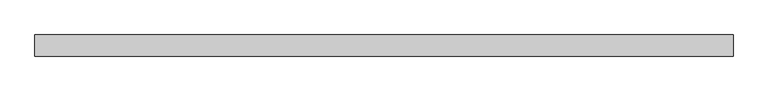
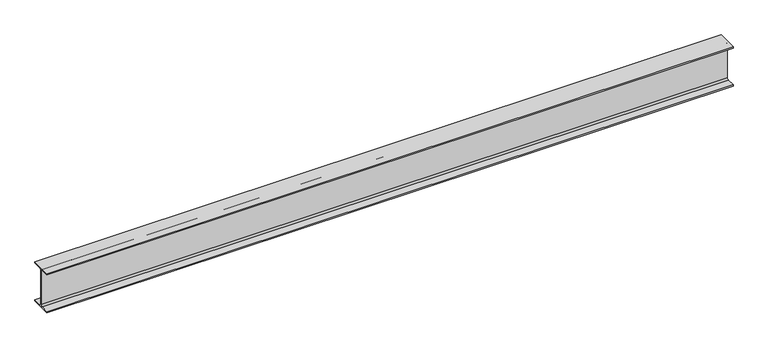
"""IFC4 building model written with IfcOpenShell, lengths in millimetres: beam geometry, 0912_Steel Framing_H-KSD3502 : H_SB_AR_S02_H-350x175x7x11_Platform."""

from ifc_helpers import new_model, si_unit, point, frame, frame_2d, origin, place, context, project, spatial, polyline, circle_curve, trimmed, segment, composite_curve, outline, extrude, source, transform, mapped, element, save


def beam_3a5a8fac(model_context):
    return source(origin(), model_context, "Body", "SweptSolid", [
        extrude(outline(composite_curve([segment(polyline([(87.5, -164.0), (87.5, -175.0), (-87.5, -175.0), (-87.5, -164.0), (-17.5, -164.0)]), True, "CONTINUOUS"), segment(trimmed(circle_curve(frame_2d((-17.5, -150.0)), 14.0), [point((-17.5, -164.0))], [point((-3.5, -150.0))], True, "CARTESIAN"), True, "CONTINUOUS"), segment(polyline([(-3.5, -150.0), (-3.5, 150.0)]), True, "CONTINUOUS"), segment(trimmed(circle_curve(frame_2d((-17.5, 150.0)), 14.0), [point((-3.5, 150.0))], [point((-17.5, 164.0))], True, "CARTESIAN"), True, "CONTINUOUS"), segment(polyline([(-17.5, 164.0), (-87.5, 164.0), (-87.5, 175.0), (87.5, 175.0), (87.5, 164.0), (17.5, 164.0)]), True, "CONTINUOUS"), segment(trimmed(circle_curve(frame_2d((17.5, 150.0)), 14.0), [point((17.5, 164.0))], [point((3.5, 150.0))], True, "CARTESIAN"), True, "CONTINUOUS"), segment(polyline([(3.5, 150.0), (3.5, -150.0)]), True, "CONTINUOUS"), segment(trimmed(circle_curve(frame_2d((17.5, -150.0)), 14.0), [point((3.5, -150.0))], [point((17.5, -164.0))], True, "CARTESIAN"), True, "CONTINUOUS"), segment(polyline([(17.5, -164.0), (87.5, -164.0)]), True, "CONTINUOUS")], self_intersect=False)), frame((-2887.3, 0.0, 0.0), z_axis=(1.0, 0.0, 0.0), x_axis=(0.0, 1.0, 0.0)), (0.0, 0.0, 1.0), 5774.6),
    ])


if __name__ == "__main__":
    model = new_model("IFC4")
    model_context = context("Model", 3, world=origin())
    ifc_project = project(units=[si_unit("LENGTHUNIT", "METRE", prefix="MILLI")], contexts=[model_context])
    site = spatial("IfcSite", under=ifc_project)
    building = spatial("IfcBuilding", under=site)
    placement = place(None, origin())
    beam_shape = beam_3a5a8fac(model_context)
    element("IfcBeam", 1, ObjectType="0912_Steel Framing_H-KSD3502 : H_SB_AR_S02_H-350x175x7x11_Platform", at=placement, inside=building, context=model_context, shape_type="MappedRepresentation", body=[
        mapped(beam_shape, transform((0.0, 0.0, 0.0), x_axis=(1.0, 0.0, 0.0), y_axis=(0.0, 1.0, 0.0), z_axis=(0.0, 0.0, 1.0))),
    ])
    save(model, "model.ifc")

# Revit data of these elements
# Type "0912_Steel Framing_H-KSD3502 : H_SB_AR_S02_H-350x175x7x11_Platform"
#   H_Q'ty Cal Type Tag = "SB-Q2"
#   H_WM Code_1 = "S01AA073-00001 |  | TON | Main Steel Structure Fabrication Work | Shelter/Building | Medium Steel - Standard |  |  |  |  |  |  | Material: (   ) | (90)KG/M>Weight≥(30)KG/M | S01AA073-00001 Main Steel Structure Fabrication Work Shelter/Building Medium Steel - Standard         | - Material: ( ASTM A36 )\n- (90)KG/M>Weight≥(30)KG/M"
#   H_WM Code_2 = "S03AA083-00001 |  | TON | Main Steel Structure Erection Work | Shelter/Building | Medium Steel |  |  |  |  |  |  | Material: (   ) | S03AA083-00001 Main Steel Structure Erection Work Shelter/Building Medium Steel         | - Material: ( ASTM A36 )"
#   H_WM Code_3 = "S01AA009-00001 |  | TON | Main Steel Structure Fabrication Work | Shelter/Building | Plates - Gusset, Stiffener, ETC | Material: (   ) | S01AA009-00001 Main Steel Structure Fabrication Work Shelter/Building Plates - Gusset, Stiffener, ETC         |"
#   H_WM Code_4 = "S41AA051-00001 |  | M2 | Steel Structure Paint Work | Shelter/Building | for Non-Fireproofed Steel Surface |  |  |  |  |  |  | Material: (   ) | S41AA051-00001 Steel Structure Paint Work Shelter/Building for Non-Fireproofed Steel Surface         |"
#   Width = 17.5 cm
#   Web Thickness = 0.7 cm
#   Web Fillet = 1.4 cm
#   Warping Constant = 282000.0 cm⁶
#   W = 0
#   Torsional Moment of Inertia = 19.4042 cm⁴
#   Section Area = 63.14 cm²
#   Plastic Modulus weak axis = 174.0 cm³
#   Plastic Modulus strong axis = 868.0 cm³
#   Perimeter = 1.36 m²/m
#   Nominal Weight = 49.60 kgf/m
#   Moment of Inertia weak axis = 984.00 cm⁴
#   Moment of Inertia strong axis = 13600.00 cm⁴
#   Height = 35.0 cm
#   Flange Thickness = 1.1 cm
#   Elastic Modulus weak axis = 112.0 cm³
#   Elastic Modulus strong axis = 775.0 cm³
#   Centroid Vertical = 17.5 cm
#   Centroid Horizontal = 8.75 cm
#   Ix = 136000000
#   Length [instance default] = 1524 mm
#   Zx = 868000
#   b = 175 mm
#   h = 350 mm
#   r = 14 mm
#   s = 7 mm
#   t = 11 mm
#   A = 0.006314 m²
#   Structural Material [instance default] = Steel, 45-345
#   Assembly Code = ""
# Element 1 (IfcBeam, "0912_Steel Framing_H-KSD3502 : H_SB_AR_S02_H-350x175x7x11_Platform")
#   Materials on its faces: "Steel, 45-345"
# Materials
#   "Steel, 45-345": class "Metal", colour RGB 189 187 185, transparency 0, Description = "Steel 345 MPa", Cost = 0
